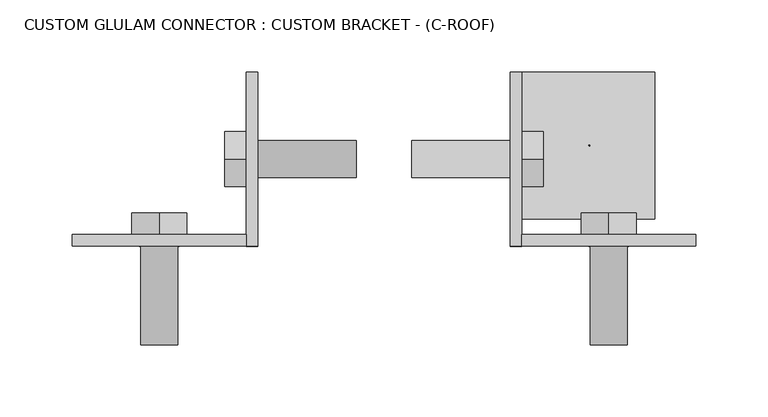
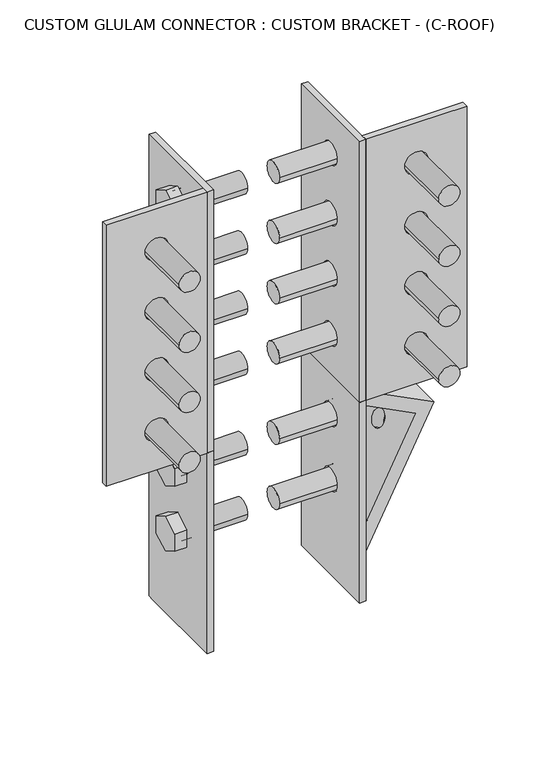
"""IFC4 building model written with IfcOpenShell, lengths in millimetres: fastener geometry, CUSTOM GLULAM CONNECTOR : CUSTOM BRACKET - (C-ROOF)."""

from ifc_helpers import new_model, si_unit, point, frame, frame_2d, origin, place, context, project, spatial, polyline, circle_curve, trimmed, segment, composite_curve, outline, extrude, source, transform, mapped, element, save
from ifc_brep_helpers import plane_surface, revolved_surface, advanced_brep


def custom_glulam_connector_custom_bracket_c_roof_8839ad80(model_context):
    return source(origin(), model_context, "Body", "SolidModel", [
        advanced_brep(
        [(-95.25, -60.325, 7.9375), (-87.3125, -60.325, 7.9375), (-87.3125, -60.325, 261.9375), (-95.25, -60.325, 261.9375), (-95.25, 60.325, 261.9375), (-87.3125, 60.325, 261.9375), (-87.3125, 60.325, 7.9375), (-95.25, 60.325, 7.9375), (-95.25, -13.890625, 128.5875), (-95.25, 13.890625, 128.5875), (-87.3125, 13.890625, 128.5875), (-87.3125, -13.890625, 128.5875), (-95.25, 52.3875, 7.9375), (-95.25, 52.3875, 261.9375), (-95.25, 13.890625, 211.1375), (-95.25, -13.890625, 211.1375), (-87.3125, -13.890625, 211.1375), (-87.3125, 13.890625, 211.1375)],
        [
            (0, 1),
            (1, 2),
            (2, 3),
            (3, 0),
            (4, 5),
            (5, 6),
            (6, 7),
            (7, 4),
            (8, 9, circle_curve(frame((-95.25, 0.0, 128.5875), z_axis=(-1.0, 0.0, 0.0), x_axis=(0.0, 1.0, 0.0)), 13.890625)),
            (9, 10),
            (10, 11, circle_curve(frame((-87.3125, 0.0, 128.5875), z_axis=(1.0, 0.0, 0.0), x_axis=(0.0, 1.0, 0.0)), 13.890625)),
            (11, 8),
            (7, 12),
            (12, 0),
            (3, 13),
            (13, 4),
            (8, 9, circle_curve(frame((-95.25, 0.0, 128.5875), z_axis=(1.0, 0.0, 0.0), x_axis=(0.0, 1.0, 0.0)), 13.890625)),
            (14, 15, circle_curve(frame((-95.25, 0.0, 211.1375), z_axis=(1.0, 0.0, 0.0), x_axis=(0.0, 1.0, 0.0)), 13.890625)),
            (15, 14, circle_curve(frame((-95.25, 0.0, 211.1375), z_axis=(1.0, 0.0, 0.0), x_axis=(0.0, 1.0, 0.0)), 13.890625)),
            (16, 17, circle_curve(frame((-87.3125, 0.0, 211.1375), z_axis=(1.0, 0.0, 0.0), x_axis=(0.0, 1.0, 0.0)), 13.890625)),
            (17, 14),
            (15, 16),
            (17, 16, circle_curve(frame((-87.3125, 0.0, 211.1375), z_axis=(1.0, 0.0, 0.0), x_axis=(0.0, 1.0, 0.0)), 13.890625)),
            (11, 10, circle_curve(frame((-87.3125, 0.0, 128.5875), z_axis=(1.0, 0.0, 0.0), x_axis=(0.0, 1.0, 0.0)), 13.890625)),
            (5, 2),
            (1, 6),
        ],
        [
            plane_surface(frame((-95.25, -60.325, 261.9375), z_axis=(0.0, -1.0, 0.0), x_axis=(1.0, 0.0, 0.0))),
            plane_surface(frame((-95.25, 60.325, 7.9375), z_axis=(0.0, 1.0, 0.0), x_axis=(1.0, 0.0, 0.0))),
            revolved_surface(polyline([(-95.25, 13.890625, 128.5875), (-87.3125, 13.890625, 128.5875)]), (-87.3125, 0.0, 128.5875), (-1.0, 0.0, 0.0)),
            plane_surface(frame((-95.25, -60.325, 261.9375), z_axis=(-1.0, 0.0, 0.0), x_axis=(0.0, -1.0, 0.0))),
            revolved_surface(polyline([(-95.25, 13.890625, 211.1375), (-87.3125, 13.890625, 211.1375)]), (-87.3125, 0.0, 211.1375), (-1.0, 0.0, 0.0)),
            plane_surface(frame((-87.3125, -60.325, 261.9375), z_axis=(1.0, 0.0, 0.0), x_axis=(0.0, 1.0, 0.0))),
            plane_surface(frame((-95.25, 60.325, 261.9375), z_axis=(0.0, 0.0, 1.0), x_axis=(1.0, 0.0, 0.0))),
            plane_surface(frame((-95.25, -60.325, 7.9375), z_axis=(0.0, 0.0, -1.0), x_axis=(1.0, 0.0, 0.0))),
        ],
        [
            (0, [[1, 2, 3, 4]]),
            (1, [[5, 6, 7, 8]]),
            (2, [[9, 10, 11, 12]]),
            (3, [[-8, 13, 14, -4, 15, 16], [-9, 17], [18, 19]]),
            (4, [[20, 21, -19, 22]]),
            (4, [[-18, -21, 23, -22]]),
            (2, [[24, -10, -17, -12]]),
            (5, [[25, -2, 26, -6], [-23, -20], [-11, -24]]),
            (6, [[-3, -25, -5, -16, -15]]),
            (7, [[-7, -26, -1, -14, -13]]),
        ],
    ),
        extrude(outline(polyline([(-19.05, 222.1360226), (0.0, 233.1345453), (19.05, 222.1360226), (19.05, 200.1389774), (0.0, 189.1404547), (-19.05, 200.1389774), (-19.05, 222.1360226)])), frame((-110.2320312, 0.0, 0.0), z_axis=(1.0, 0.0, 0.0), x_axis=(0.0, 1.0, 0.0)), (0.0, 0.0, 1.0), 14.9820312),
        extrude(outline(composite_curve([segment(trimmed(circle_curve(frame_2d((0.0, 211.1375)), 12.7), [point((-12.7, 211.1375))], [point((12.7, 211.1375))], False, "CARTESIAN"), True, "CONTINUOUS"), segment(trimmed(circle_curve(frame_2d((0.0, 211.1375)), 12.7), [point((12.7, 211.1375))], [point((-12.7, 211.1375))], False, "CARTESIAN"), True, "CONTINUOUS")], self_intersect=False)), frame((-95.25, 0.0, 0.0), z_axis=(1.0, 0.0, 0.0), x_axis=(0.0, 1.0, 0.0)), (0.0, 0.0, 1.0), 76.2),
        extrude(outline(polyline([(-19.05, 139.5860226), (0.0, 150.5845453), (19.05, 139.5860226), (19.05, 117.5889774), (0.0, 106.5904547), (-19.05, 117.5889774), (-19.05, 139.5860226)])), frame((-110.2320312, 0.0, 0.0), z_axis=(1.0, 0.0, 0.0), x_axis=(0.0, 1.0, 0.0)), (0.0, 0.0, 1.0), 14.9820312),
        extrude(outline(composite_curve([segment(trimmed(circle_curve(frame_2d((0.0, 128.5875)), 12.7), [point((-12.7, 128.5875))], [point((12.7, 128.5875))], False, "CARTESIAN"), True, "CONTINUOUS"), segment(trimmed(circle_curve(frame_2d((0.0, 128.5875)), 12.7), [point((12.7, 128.5875))], [point((-12.7, 128.5875))], False, "CARTESIAN"), True, "CONTINUOUS")], self_intersect=False)), frame((-95.25, 0.0, 0.0), z_axis=(1.0, 0.0, 0.0), x_axis=(0.0, 1.0, 0.0)), (0.0, 0.0, 1.0), 76.2),
        extrude(outline(polyline([(-19.05, 222.1360226), (0.0, 233.1345453), (19.05, 222.1360226), (19.05, 200.1389774), (0.0, 189.1404547), (-19.05, 200.1389774), (-19.05, 222.1360226)])), frame((-110.2320312, 0.0, 0.0), z_axis=(1.0, 0.0, 0.0), x_axis=(0.0, 1.0, 0.0)), (0.0, 0.0, 1.0), 14.9820312),
        extrude(outline(composite_curve([segment(trimmed(circle_curve(frame_2d((0.0, 211.1375)), 12.7), [point((-12.7, 211.1375))], [point((12.7, 211.1375))], False, "CARTESIAN"), True, "CONTINUOUS"), segment(trimmed(circle_curve(frame_2d((0.0, 211.1375)), 12.7), [point((12.7, 211.1375))], [point((-12.7, 211.1375))], False, "CARTESIAN"), True, "CONTINUOUS")], self_intersect=False)), frame((-95.25, 0.0, 0.0), z_axis=(1.0, 0.0, 0.0), x_axis=(0.0, 1.0, 0.0)), (0.0, 0.0, 1.0), 76.2),
        advanced_brep(
        [(95.25, -60.325, 7.9375), (95.25, -60.325, 261.9375), (87.3125, -60.325, 261.9375), (87.3125, -60.325, 7.9375), (95.25, 60.325, 261.9375), (95.25, 60.325, 7.9375), (87.3125, 60.325, 7.9375), (87.3125, 60.325, 261.9375), (95.25, -13.890625, 128.5875), (87.3125, -13.890625, 128.5875), (87.3125, 13.890625, 128.5875), (95.25, 13.890625, 128.5875), (95.25, 52.3875, 261.9375), (95.25, 52.3875, 7.9375), (95.25, 13.890625, 211.1375), (95.25, -13.890625, 211.1375), (87.3125, -13.890625, 211.1375), (87.3125, 13.890625, 211.1375)],
        [
            (0, 1),
            (1, 2),
            (2, 3),
            (3, 0),
            (4, 5),
            (5, 6),
            (6, 7),
            (7, 4),
            (8, 9),
            (9, 10, circle_curve(frame((87.3125, 0.0, 128.5875), z_axis=(-1.0, 0.0, 0.0), x_axis=(0.0, 1.0, 0.0)), 13.890625)),
            (10, 11),
            (11, 8, circle_curve(frame((95.25, 0.0, 128.5875), z_axis=(1.0, 0.0, 0.0), x_axis=(0.0, 1.0, 0.0)), 13.890625)),
            (4, 12),
            (12, 1),
            (0, 13),
            (13, 5),
            (14, 15, circle_curve(frame((95.25, 0.0, 211.1375), z_axis=(-1.0, 0.0, 0.0), x_axis=(0.0, 1.0, 0.0)), 13.890625)),
            (15, 14, circle_curve(frame((95.25, 0.0, 211.1375), z_axis=(-1.0, 0.0, 0.0), x_axis=(0.0, 1.0, 0.0)), 13.890625)),
            (11, 8, circle_curve(frame((95.25, 0.0, 128.5875), z_axis=(-1.0, 0.0, 0.0), x_axis=(0.0, 1.0, 0.0)), 13.890625)),
            (16, 15),
            (14, 17),
            (17, 16, circle_curve(frame((87.3125, 0.0, 211.1375), z_axis=(-1.0, 0.0, 0.0), x_axis=(0.0, 1.0, 0.0)), 13.890625)),
            (16, 17, circle_curve(frame((87.3125, 0.0, 211.1375), z_axis=(-1.0, 0.0, 0.0), x_axis=(0.0, 1.0, 0.0)), 13.890625)),
            (10, 9, circle_curve(frame((87.3125, 0.0, 128.5875), z_axis=(-1.0, 0.0, 0.0), x_axis=(0.0, 1.0, 0.0)), 13.890625)),
            (6, 3),
            (2, 7),
        ],
        [
            plane_surface(frame((95.25, -60.325, 261.9375), z_axis=(0.0, -1.0, 0.0), x_axis=(-1.0, 0.0, 0.0))),
            plane_surface(frame((95.25, 60.325, 7.9375), z_axis=(0.0, 1.0, 0.0), x_axis=(-1.0, 0.0, 0.0))),
            revolved_surface(polyline([(95.25, 13.890625, 128.5875), (87.3125, 13.890625, 128.5875)]), (87.3125, 0.0, 128.5875), (1.0, 0.0, 0.0)),
            plane_surface(frame((95.25, -60.325, 261.9375), z_axis=(1.0, 0.0, 0.0), x_axis=(0.0, -1.0, 0.0))),
            revolved_surface(polyline([(95.25, 13.890625, 211.1375), (87.3125, 13.890625, 211.1375)]), (87.3125, 0.0, 211.1375), (1.0, 0.0, 0.0)),
            plane_surface(frame((87.3125, -60.325, 261.9375), z_axis=(-1.0, 0.0, 0.0), x_axis=(0.0, 1.0, 0.0))),
            plane_surface(frame((95.25, 60.325, 261.9375), z_axis=(0.0, 0.0, 1.0), x_axis=(-1.0, 0.0, 0.0))),
            plane_surface(frame((95.25, -60.325, 7.9375), z_axis=(0.0, 0.0, -1.0), x_axis=(-1.0, 0.0, 0.0))),
        ],
        [
            (0, [[1, 2, 3, 4]]),
            (1, [[5, 6, 7, 8]]),
            (2, [[9, 10, 11, 12]]),
            (3, [[13, 14, -1, 15, 16, -5], [17, 18], [19, -12]]),
            (4, [[20, -17, 21, 22]]),
            (4, [[-20, 23, -21, -18]]),
            (2, [[-9, -19, -11, 24]]),
            (5, [[-7, 25, -3, 26], [-22, -23], [-24, -10]]),
            (6, [[-14, -13, -8, -26, -2]]),
            (7, [[-16, -15, -4, -25, -6]]),
        ],
    ),
        extrude(outline(polyline([(-19.05, 222.1360226), (0.0, 233.1345453), (19.05, 222.1360226), (19.05, 200.1389774), (0.0, 189.1404547), (-19.05, 200.1389774), (-19.05, 222.1360226)])), frame((95.25, 0.0, 0.0), z_axis=(1.0, 0.0, 0.0), x_axis=(0.0, 1.0, 0.0)), (0.0, 0.0, 1.0), 14.9820312),
        extrude(outline(composite_curve([segment(trimmed(circle_curve(frame_2d((0.0, 211.1375)), 12.7), [point((-12.7, 211.1375))], [point((12.7, 211.1375))], False, "CARTESIAN"), True, "CONTINUOUS"), segment(trimmed(circle_curve(frame_2d((0.0, 211.1375)), 12.7), [point((12.7, 211.1375))], [point((-12.7, 211.1375))], False, "CARTESIAN"), True, "CONTINUOUS")], self_intersect=False)), frame((19.05, 0.0, 0.0), z_axis=(1.0, 0.0, 0.0), x_axis=(0.0, 1.0, 0.0)), (0.0, 0.0, 1.0), 76.2),
        extrude(outline(polyline([(-19.05, 139.5860226), (0.0, 150.5845453), (19.05, 139.5860226), (19.05, 117.5889774), (0.0, 106.5904547), (-19.05, 117.5889774), (-19.05, 139.5860226)])), frame((95.25, 0.0, 0.0), z_axis=(1.0, 0.0, 0.0), x_axis=(0.0, 1.0, 0.0)), (0.0, 0.0, 1.0), 14.9820312),
        extrude(outline(composite_curve([segment(trimmed(circle_curve(frame_2d((0.0, 128.5875)), 12.7), [point((-12.7, 128.5875))], [point((12.7, 128.5875))], False, "CARTESIAN"), True, "CONTINUOUS"), segment(trimmed(circle_curve(frame_2d((0.0, 128.5875)), 12.7), [point((12.7, 128.5875))], [point((-12.7, 128.5875))], False, "CARTESIAN"), True, "CONTINUOUS")], self_intersect=False)), frame((19.05, 0.0, 0.0), z_axis=(1.0, 0.0, 0.0), x_axis=(0.0, 1.0, 0.0)), (0.0, 0.0, 1.0), 76.2),
        extrude(outline(polyline([(-19.05, 222.1360226), (0.0, 233.1345453), (19.05, 222.1360226), (19.05, 200.1389774), (0.0, 189.1404547), (-19.05, 200.1389774), (-19.05, 222.1360226)])), frame((95.25, 0.0, 0.0), z_axis=(1.0, 0.0, 0.0), x_axis=(0.0, 1.0, 0.0)), (0.0, 0.0, 1.0), 14.9820312),
        extrude(outline(composite_curve([segment(trimmed(circle_curve(frame_2d((0.0, 211.1375)), 12.7), [point((-12.7, 211.1375))], [point((12.7, 211.1375))], False, "CARTESIAN"), True, "CONTINUOUS"), segment(trimmed(circle_curve(frame_2d((0.0, 211.1375)), 12.7), [point((12.7, 211.1375))], [point((-12.7, 211.1375))], False, "CARTESIAN"), True, "CONTINUOUS")], self_intersect=False)), frame((19.05, 0.0, 0.0), z_axis=(1.0, 0.0, 0.0), x_axis=(0.0, 1.0, 0.0)), (0.0, 0.0, 1.0), 76.2),
        extrude(outline(polyline([(592.1375, -215.9), (261.9375, -215.9), (261.9375, -95.25), (592.1375, -95.25), (592.1375, -215.9)]), holes=[composite_curve([segment(trimmed(circle_curve(frame_2d((541.3375, -155.575)), 13.890625), [point((541.3375, -141.684375))], [point((541.3375, -169.465625))], True, "CARTESIAN"), True, "CONTINUOUS"), segment(trimmed(circle_curve(frame_2d((541.3375, -155.575)), 13.890625), [point((541.3375, -169.465625))], [point((541.3375, -141.684375))], True, "CARTESIAN"), True, "CONTINUOUS")], self_intersect=False), composite_curve([segment(trimmed(circle_curve(frame_2d((465.1375, -155.575)), 13.890625), [point((465.1375, -141.684375))], [point((465.1375, -169.465625))], True, "CARTESIAN"), True, "CONTINUOUS"), segment(trimmed(circle_curve(frame_2d((465.1375, -155.575)), 13.890625), [point((465.1375, -169.465625))], [point((465.1375, -141.684375))], True, "CARTESIAN"), True, "CONTINUOUS")], self_intersect=False), composite_curve([segment(trimmed(circle_curve(frame_2d((388.9375, -155.575)), 13.890625), [point((388.9375, -141.684375))], [point((388.9375, -169.465625))], True, "CARTESIAN"), True, "CONTINUOUS"), segment(trimmed(circle_curve(frame_2d((388.9375, -155.575)), 13.890625), [point((388.9375, -169.465625))], [point((388.9375, -141.684375))], True, "CARTESIAN"), True, "CONTINUOUS")], self_intersect=False), composite_curve([segment(trimmed(circle_curve(frame_2d((312.7375, -155.575)), 13.890625), [point((312.7375, -141.684375))], [point((312.7375, -169.465625))], True, "CARTESIAN"), True, "CONTINUOUS"), segment(trimmed(circle_curve(frame_2d((312.7375, -155.575)), 13.890625), [point((312.7375, -169.465625))], [point((312.7375, -141.684375))], True, "CARTESIAN"), True, "CONTINUOUS")], self_intersect=False)]), frame((0.0, -60.325, 0.0), z_axis=(0.0, 1.0, 0.0), x_axis=(0.0, 0.0, 1.0)), (0.0, 0.0, 1.0), 7.9375),
        extrude(outline(polyline([(552.3360226, -136.525), (563.3345453, -155.575), (552.3360226, -174.625), (530.3389774, -174.625), (519.3404547, -155.575), (530.3389774, -136.525), (552.3360226, -136.525)])), frame((0.0, -52.3875, 0.0), z_axis=(0.0, 1.0, 0.0), x_axis=(0.0, 0.0, 1.0)), (0.0, 0.0, 1.0), 14.9820312),
        extrude(outline(composite_curve([segment(trimmed(circle_curve(frame_2d((541.3375, -155.575)), 12.7), [point((541.3375, -142.875))], [point((541.3375, -168.275))], False, "CARTESIAN"), True, "CONTINUOUS"), segment(trimmed(circle_curve(frame_2d((541.3375, -155.575)), 12.7), [point((541.3375, -168.275))], [point((541.3375, -142.875))], False, "CARTESIAN"), True, "CONTINUOUS")], self_intersect=False)), frame((0.0, -128.5875, 0.0), z_axis=(0.0, 1.0, 0.0), x_axis=(0.0, 0.0, 1.0)), (0.0, 0.0, 1.0), 76.2),
        extrude(outline(polyline([(476.1360226, -136.525), (487.1345453, -155.575), (476.1360226, -174.625), (454.1389774, -174.625), (443.1404547, -155.575), (454.1389774, -136.525), (476.1360226, -136.525)])), frame((0.0, -52.3875, 0.0), z_axis=(0.0, 1.0, 0.0), x_axis=(0.0, 0.0, 1.0)), (0.0, 0.0, 1.0), 14.9820312),
        extrude(outline(composite_curve([segment(trimmed(circle_curve(frame_2d((465.1375, -155.575)), 12.7), [point((465.1375, -142.875))], [point((465.1375, -168.275))], False, "CARTESIAN"), True, "CONTINUOUS"), segment(trimmed(circle_curve(frame_2d((465.1375, -155.575)), 12.7), [point((465.1375, -168.275))], [point((465.1375, -142.875))], False, "CARTESIAN"), True, "CONTINUOUS")], self_intersect=False)), frame((0.0, -128.5875, 0.0), z_axis=(0.0, 1.0, 0.0), x_axis=(0.0, 0.0, 1.0)), (0.0, 0.0, 1.0), 76.2),
        extrude(outline(polyline([(552.3360226, -136.525), (563.3345453, -155.575), (552.3360226, -174.625), (530.3389774, -174.625), (519.3404547, -155.575), (530.3389774, -136.525), (552.3360226, -136.525)])), frame((0.0, -52.3875, 0.0), z_axis=(0.0, 1.0, 0.0), x_axis=(0.0, 0.0, 1.0)), (0.0, 0.0, 1.0), 14.9820312),
        extrude(outline(composite_curve([segment(trimmed(circle_curve(frame_2d((541.3375, -155.575)), 12.7), [point((541.3375, -142.875))], [point((541.3375, -168.275))], False, "CARTESIAN"), True, "CONTINUOUS"), segment(trimmed(circle_curve(frame_2d((541.3375, -155.575)), 12.7), [point((541.3375, -168.275))], [point((541.3375, -142.875))], False, "CARTESIAN"), True, "CONTINUOUS")], self_intersect=False)), frame((0.0, -128.5875, 0.0), z_axis=(0.0, 1.0, 0.0), x_axis=(0.0, 0.0, 1.0)), (0.0, 0.0, 1.0), 76.2),
        extrude(outline(polyline([(399.9360226, -136.525), (410.9345453, -155.575), (399.9360226, -174.625), (377.9389774, -174.625), (366.9404547, -155.575), (377.9389774, -136.525), (399.9360226, -136.525)])), frame((0.0, -52.3875, 0.0), z_axis=(0.0, 1.0, 0.0), x_axis=(0.0, 0.0, 1.0)), (0.0, 0.0, 1.0), 14.9820312),
        extrude(outline(composite_curve([segment(trimmed(circle_curve(frame_2d((388.9375, -155.575)), 12.7), [point((388.9375, -142.875))], [point((388.9375, -168.275))], False, "CARTESIAN"), True, "CONTINUOUS"), segment(trimmed(circle_curve(frame_2d((388.9375, -155.575)), 12.7), [point((388.9375, -168.275))], [point((388.9375, -142.875))], False, "CARTESIAN"), True, "CONTINUOUS")], self_intersect=False)), frame((0.0, -128.5875, 0.0), z_axis=(0.0, 1.0, 0.0), x_axis=(0.0, 0.0, 1.0)), (0.0, 0.0, 1.0), 76.2),
        extrude(outline(polyline([(323.7360226, -136.525), (334.7345453, -155.575), (323.7360226, -174.625), (301.7389774, -174.625), (290.7404547, -155.575), (301.7389774, -136.525), (323.7360226, -136.525)])), frame((0.0, -52.3875, 0.0), z_axis=(0.0, 1.0, 0.0), x_axis=(0.0, 0.0, 1.0)), (0.0, 0.0, 1.0), 14.9820312),
        extrude(outline(composite_curve([segment(trimmed(circle_curve(frame_2d((312.7375, -155.575)), 12.7), [point((312.7375, -142.875))], [point((312.7375, -168.275))], False, "CARTESIAN"), True, "CONTINUOUS"), segment(trimmed(circle_curve(frame_2d((312.7375, -155.575)), 12.7), [point((312.7375, -168.275))], [point((312.7375, -142.875))], False, "CARTESIAN"), True, "CONTINUOUS")], self_intersect=False)), frame((0.0, -128.5875, 0.0), z_axis=(0.0, 1.0, 0.0), x_axis=(0.0, 0.0, 1.0)), (0.0, 0.0, 1.0), 76.2),
        advanced_brep(
        [(-95.25, -60.325, 261.9375), (-87.3125, -60.325, 261.9375), (-87.3125, -60.325, 592.1375), (-95.25, -60.325, 592.1375), (-95.25, 60.325, 592.1375), (-87.3125, 60.325, 592.1375), (-87.3125, 60.325, 261.9375), (-95.25, 60.325, 261.9375), (-95.25, -13.890625, 465.1375), (-95.25, 13.890625, 465.1375), (-87.3125, 13.890625, 465.1375), (-87.3125, -13.890625, 465.1375), (-95.25, -52.3875, 261.9375), (-95.25, -52.3875, 592.1375), (-95.25, 13.890625, 541.3375), (-95.25, -13.890625, 541.3375), (-95.25, 13.890625, 388.9375), (-95.25, -13.890625, 388.9375), (-95.25, 13.890625, 312.7375), (-95.25, -13.890625, 312.7375), (-87.3125, -13.890625, 541.3375), (-87.3125, 13.890625, 541.3375), (-87.3125, -13.890625, 388.9375), (-87.3125, 13.890625, 388.9375), (-87.3125, -13.890625, 312.7375), (-87.3125, 13.890625, 312.7375)],
        [
            (0, 1),
            (1, 2),
            (2, 3),
            (3, 0),
            (4, 5),
            (5, 6),
            (6, 7),
            (7, 4),
            (8, 9, circle_curve(frame((-95.25, 0.0, 465.1375), z_axis=(-1.0, 0.0, 0.0), x_axis=(0.0, 1.0, 0.0)), 13.890625)),
            (9, 10),
            (10, 11, circle_curve(frame((-87.3125, 0.0, 465.1375), z_axis=(1.0, 0.0, 0.0), x_axis=(0.0, 1.0, 0.0)), 13.890625)),
            (11, 8),
            (7, 12),
            (12, 0),
            (3, 13),
            (13, 4),
            (8, 9, circle_curve(frame((-95.25, 0.0, 465.1375), z_axis=(1.0, 0.0, 0.0), x_axis=(0.0, 1.0, 0.0)), 13.890625)),
            (14, 15, circle_curve(frame((-95.25, 0.0, 541.3375), z_axis=(1.0, 0.0, 0.0), x_axis=(0.0, 1.0, 0.0)), 13.890625)),
            (15, 14, circle_curve(frame((-95.25, 0.0, 541.3375), z_axis=(1.0, 0.0, 0.0), x_axis=(0.0, 1.0, 0.0)), 13.890625)),
            (16, 17, circle_curve(frame((-95.25, 0.0, 388.9375), z_axis=(1.0, 0.0, 0.0), x_axis=(0.0, 1.0, 0.0)), 13.890625)),
            (17, 16, circle_curve(frame((-95.25, 0.0, 388.9375), z_axis=(1.0, 0.0, 0.0), x_axis=(0.0, 1.0, 0.0)), 13.890625)),
            (18, 19, circle_curve(frame((-95.25, 0.0, 312.7375), z_axis=(1.0, 0.0, 0.0), x_axis=(0.0, 1.0, 0.0)), 13.890625)),
            (19, 18, circle_curve(frame((-95.25, 0.0, 312.7375), z_axis=(1.0, 0.0, 0.0), x_axis=(0.0, 1.0, 0.0)), 13.890625)),
            (20, 21, circle_curve(frame((-87.3125, 0.0, 541.3375), z_axis=(1.0, 0.0, 0.0), x_axis=(0.0, 1.0, 0.0)), 13.890625)),
            (21, 14),
            (15, 20),
            (21, 20, circle_curve(frame((-87.3125, 0.0, 541.3375), z_axis=(1.0, 0.0, 0.0), x_axis=(0.0, 1.0, 0.0)), 13.890625)),
            (11, 10, circle_curve(frame((-87.3125, 0.0, 465.1375), z_axis=(1.0, 0.0, 0.0), x_axis=(0.0, 1.0, 0.0)), 13.890625)),
            (5, 2),
            (1, 6),
            (22, 23, circle_curve(frame((-87.3125, 0.0, 388.9375), z_axis=(-1.0, 0.0, 0.0), x_axis=(0.0, 1.0, 0.0)), 13.890625)),
            (23, 22, circle_curve(frame((-87.3125, 0.0, 388.9375), z_axis=(-1.0, 0.0, 0.0), x_axis=(0.0, 1.0, 0.0)), 13.890625)),
            (24, 25, circle_curve(frame((-87.3125, 0.0, 312.7375), z_axis=(-1.0, 0.0, 0.0), x_axis=(0.0, 1.0, 0.0)), 13.890625)),
            (25, 24, circle_curve(frame((-87.3125, 0.0, 312.7375), z_axis=(-1.0, 0.0, 0.0), x_axis=(0.0, 1.0, 0.0)), 13.890625)),
            (18, 25),
            (24, 19),
            (16, 23),
            (22, 17),
        ],
        [
            plane_surface(frame((-95.25, -60.325, 592.1375), z_axis=(0.0, -1.0, 0.0), x_axis=(1.0, 0.0, 0.0))),
            plane_surface(frame((-95.25, 60.325, 261.9375), z_axis=(0.0, 1.0, 0.0), x_axis=(1.0, 0.0, 0.0))),
            revolved_surface(polyline([(-95.25, 13.890625, 465.1375), (-87.3125, 13.890625, 465.1375)]), (-87.3125, 0.0, 465.1375), (-1.0, 0.0, 0.0)),
            plane_surface(frame((-95.25, -60.325, 592.1375), z_axis=(-1.0, 0.0, 0.0), x_axis=(0.0, -1.0, 0.0))),
            revolved_surface(polyline([(-95.25, 13.890625, 541.3375), (-87.3125, 13.890625, 541.3375)]), (-87.3125, 0.0, 541.3375), (-1.0, 0.0, 0.0)),
            plane_surface(frame((-87.3125, -60.325, 592.1375), z_axis=(1.0, 0.0, 0.0), x_axis=(0.0, 1.0, 0.0))),
            plane_surface(frame((-95.25, 60.325, 592.1375), z_axis=(0.0, 0.0, 1.0), x_axis=(1.0, 0.0, 0.0))),
            plane_surface(frame((-95.25, -60.325, 261.9375), z_axis=(0.0, 0.0, -1.0), x_axis=(1.0, 0.0, 0.0))),
            revolved_surface(polyline([(-95.25, 13.890625, 312.7375), (-87.3125, 13.890625, 312.7375)]), (-87.3125, 0.0, 312.7375), (-1.0, 0.0, 0.0)),
            revolved_surface(polyline([(-95.25, 13.890625, 388.9375), (-87.3125, 13.890625, 388.9375)]), (-87.3125, 0.0, 388.9375), (-1.0, 0.0, 0.0)),
        ],
        [
            (0, [[1, 2, 3, 4]]),
            (1, [[5, 6, 7, 8]]),
            (2, [[9, 10, 11, 12]]),
            (3, [[-8, 13, 14, -4, 15, 16], [-9, 17], [18, 19], [20, 21], [22, 23]]),
            (4, [[24, 25, -19, 26]]),
            (4, [[-18, -25, 27, -26]]),
            (2, [[28, -10, -17, -12]]),
            (5, [[29, -2, 30, -6], [-27, -24], [-11, -28], [31, 32], [33, 34]]),
            (6, [[-3, -29, -5, -16, -15]]),
            (7, [[-7, -30, -1, -14, -13]]),
            (8, [[-22, 35, -33, 36]]),
            (9, [[-20, 37, -31, 38]]),
            (8, [[-34, -35, -23, -36]]),
            (9, [[-32, -37, -21, -38]]),
        ],
    ),
        extrude(outline(polyline([(-19.05, 552.3360226), (0.0, 563.3345453), (19.05, 552.3360226), (19.05, 530.3389774), (0.0, 519.3404547), (-19.05, 530.3389774), (-19.05, 552.3360226)])), frame((-110.2320312, 0.0, 0.0), z_axis=(1.0, 0.0, 0.0), x_axis=(0.0, 1.0, 0.0)), (0.0, 0.0, 1.0), 14.9820312),
        extrude(outline(composite_curve([segment(trimmed(circle_curve(frame_2d((0.0, 541.3375)), 12.7), [point((-12.7, 541.3375))], [point((12.7, 541.3375))], False, "CARTESIAN"), True, "CONTINUOUS"), segment(trimmed(circle_curve(frame_2d((0.0, 541.3375)), 12.7), [point((12.7, 541.3375))], [point((-12.7, 541.3375))], False, "CARTESIAN"), True, "CONTINUOUS")], self_intersect=False)), frame((-95.25, 0.0, 0.0), z_axis=(1.0, 0.0, 0.0), x_axis=(0.0, 1.0, 0.0)), (0.0, 0.0, 1.0), 76.2),
        extrude(outline(polyline([(-19.05, 476.1360226), (0.0, 487.1345453), (19.05, 476.1360226), (19.05, 454.1389774), (0.0, 443.1404547), (-19.05, 454.1389774), (-19.05, 476.1360226)])), frame((-110.2320312, 0.0, 0.0), z_axis=(1.0, 0.0, 0.0), x_axis=(0.0, 1.0, 0.0)), (0.0, 0.0, 1.0), 14.9820312),
        extrude(outline(composite_curve([segment(trimmed(circle_curve(frame_2d((0.0, 465.1375)), 12.7), [point((-12.7, 465.1375))], [point((12.7, 465.1375))], False, "CARTESIAN"), True, "CONTINUOUS"), segment(trimmed(circle_curve(frame_2d((0.0, 465.1375)), 12.7), [point((12.7, 465.1375))], [point((-12.7, 465.1375))], False, "CARTESIAN"), True, "CONTINUOUS")], self_intersect=False)), frame((-95.25, 0.0, 0.0), z_axis=(1.0, 0.0, 0.0), x_axis=(0.0, 1.0, 0.0)), (0.0, 0.0, 1.0), 76.2),
        extrude(outline(polyline([(-19.05, 552.3360226), (0.0, 563.3345453), (19.05, 552.3360226), (19.05, 530.3389774), (0.0, 519.3404547), (-19.05, 530.3389774), (-19.05, 552.3360226)])), frame((-110.2320312, 0.0, 0.0), z_axis=(1.0, 0.0, 0.0), x_axis=(0.0, 1.0, 0.0)), (0.0, 0.0, 1.0), 14.9820312),
        extrude(outline(composite_curve([segment(trimmed(circle_curve(frame_2d((0.0, 541.3375)), 12.7), [point((-12.7, 541.3375))], [point((12.7, 541.3375))], False, "CARTESIAN"), True, "CONTINUOUS"), segment(trimmed(circle_curve(frame_2d((0.0, 541.3375)), 12.7), [point((12.7, 541.3375))], [point((-12.7, 541.3375))], False, "CARTESIAN"), True, "CONTINUOUS")], self_intersect=False)), frame((-95.25, 0.0, 0.0), z_axis=(1.0, 0.0, 0.0), x_axis=(0.0, 1.0, 0.0)), (0.0, 0.0, 1.0), 76.2),
        extrude(outline(polyline([(-19.05, 399.9360226), (0.0, 410.9345453), (19.05, 399.9360226), (19.05, 377.9389774), (0.0, 366.9404547), (-19.05, 377.9389774), (-19.05, 399.9360226)])), frame((-110.2320312, 0.0, 0.0), z_axis=(1.0, 0.0, 0.0), x_axis=(0.0, 1.0, 0.0)), (0.0, 0.0, 1.0), 14.9820312),
        extrude(outline(composite_curve([segment(trimmed(circle_curve(frame_2d((0.0, 388.9375)), 12.7), [point((-12.7, 388.9375))], [point((12.7, 388.9375))], False, "CARTESIAN"), True, "CONTINUOUS"), segment(trimmed(circle_curve(frame_2d((0.0, 388.9375)), 12.7), [point((12.7, 388.9375))], [point((-12.7, 388.9375))], False, "CARTESIAN"), True, "CONTINUOUS")], self_intersect=False)), frame((-95.25, 0.0, 0.0), z_axis=(1.0, 0.0, 0.0), x_axis=(0.0, 1.0, 0.0)), (0.0, 0.0, 1.0), 76.2),
        extrude(outline(polyline([(-19.05, 323.7360226), (0.0, 334.7345453), (19.05, 323.7360226), (19.05, 301.7389774), (0.0, 290.7404547), (-19.05, 301.7389774), (-19.05, 323.7360226)])), frame((-110.2320312, 0.0, 0.0), z_axis=(1.0, 0.0, 0.0), x_axis=(0.0, 1.0, 0.0)), (0.0, 0.0, 1.0), 14.9820312),
        extrude(outline(composite_curve([segment(trimmed(circle_curve(frame_2d((0.0, 312.7375)), 12.7), [point((-12.7, 312.7375))], [point((12.7, 312.7375))], False, "CARTESIAN"), True, "CONTINUOUS"), segment(trimmed(circle_curve(frame_2d((0.0, 312.7375)), 12.7), [point((12.7, 312.7375))], [point((-12.7, 312.7375))], False, "CARTESIAN"), True, "CONTINUOUS")], self_intersect=False)), frame((-95.25, 0.0, 0.0), z_axis=(1.0, 0.0, 0.0), x_axis=(0.0, 1.0, 0.0)), (0.0, 0.0, 1.0), 76.2),
        extrude(outline(polyline([(592.1375, 215.9), (592.1375, 95.25), (261.9375, 95.25), (261.9375, 215.9), (592.1375, 215.9)]), holes=[composite_curve([segment(trimmed(circle_curve(frame_2d((541.3375, 155.575)), 13.890625), [point((541.3375, 141.684375))], [point((541.3375, 169.465625))], True, "CARTESIAN"), True, "CONTINUOUS"), segment(trimmed(circle_curve(frame_2d((541.3375, 155.575)), 13.890625), [point((541.3375, 169.465625))], [point((541.3375, 141.684375))], True, "CARTESIAN"), True, "CONTINUOUS")], self_intersect=False), composite_curve([segment(trimmed(circle_curve(frame_2d((465.1375, 155.575)), 13.890625), [point((465.1375, 141.684375))], [point((465.1375, 169.465625))], True, "CARTESIAN"), True, "CONTINUOUS"), segment(trimmed(circle_curve(frame_2d((465.1375, 155.575)), 13.890625), [point((465.1375, 169.465625))], [point((465.1375, 141.684375))], True, "CARTESIAN"), True, "CONTINUOUS")], self_intersect=False), composite_curve([segment(trimmed(circle_curve(frame_2d((388.9375, 155.575)), 13.890625), [point((388.9375, 141.684375))], [point((388.9375, 169.465625))], True, "CARTESIAN"), True, "CONTINUOUS"), segment(trimmed(circle_curve(frame_2d((388.9375, 155.575)), 13.890625), [point((388.9375, 169.465625))], [point((388.9375, 141.684375))], True, "CARTESIAN"), True, "CONTINUOUS")], self_intersect=False), composite_curve([segment(trimmed(circle_curve(frame_2d((312.7375, 155.575)), 13.890625), [point((312.7375, 141.684375))], [point((312.7375, 169.465625))], True, "CARTESIAN"), True, "CONTINUOUS"), segment(trimmed(circle_curve(frame_2d((312.7375, 155.575)), 13.890625), [point((312.7375, 169.465625))], [point((312.7375, 141.684375))], True, "CARTESIAN"), True, "CONTINUOUS")], self_intersect=False)]), frame((0.0, -60.325, 0.0), z_axis=(0.0, 1.0, 0.0), x_axis=(0.0, 0.0, 1.0)), (0.0, 0.0, 1.0), 7.9375),
        extrude(outline(polyline([(552.3360226, 136.525), (530.3389774, 136.525), (519.3404547, 155.575), (530.3389774, 174.625), (552.3360226, 174.625), (563.3345453, 155.575), (552.3360226, 136.525)])), frame((0.0, -52.3875, 0.0), z_axis=(0.0, 1.0, 0.0), x_axis=(0.0, 0.0, 1.0)), (0.0, 0.0, 1.0), 14.9820312),
        extrude(outline(composite_curve([segment(trimmed(circle_curve(frame_2d((541.3375, 155.575)), 12.7), [point((541.3375, 142.875))], [point((541.3375, 168.275))], False, "CARTESIAN"), True, "CONTINUOUS"), segment(trimmed(circle_curve(frame_2d((541.3375, 155.575)), 12.7), [point((541.3375, 168.275))], [point((541.3375, 142.875))], False, "CARTESIAN"), True, "CONTINUOUS")], self_intersect=False)), frame((0.0, -128.5875, 0.0), z_axis=(0.0, 1.0, 0.0), x_axis=(0.0, 0.0, 1.0)), (0.0, 0.0, 1.0), 76.2),
        extrude(outline(polyline([(476.1360226, 136.525), (454.1389774, 136.525), (443.1404547, 155.575), (454.1389774, 174.625), (476.1360226, 174.625), (487.1345453, 155.575), (476.1360226, 136.525)])), frame((0.0, -52.3875, 0.0), z_axis=(0.0, 1.0, 0.0), x_axis=(0.0, 0.0, 1.0)), (0.0, 0.0, 1.0), 14.9820312),
        extrude(outline(composite_curve([segment(trimmed(circle_curve(frame_2d((465.1375, 155.575)), 12.7), [point((465.1375, 142.875))], [point((465.1375, 168.275))], False, "CARTESIAN"), True, "CONTINUOUS"), segment(trimmed(circle_curve(frame_2d((465.1375, 155.575)), 12.7), [point((465.1375, 168.275))], [point((465.1375, 142.875))], False, "CARTESIAN"), True, "CONTINUOUS")], self_intersect=False)), frame((0.0, -128.5875, 0.0), z_axis=(0.0, 1.0, 0.0), x_axis=(0.0, 0.0, 1.0)), (0.0, 0.0, 1.0), 76.2),
        extrude(outline(polyline([(552.3360226, 136.525), (530.3389774, 136.525), (519.3404547, 155.575), (530.3389774, 174.625), (552.3360226, 174.625), (563.3345453, 155.575), (552.3360226, 136.525)])), frame((0.0, -52.3875, 0.0), z_axis=(0.0, 1.0, 0.0), x_axis=(0.0, 0.0, 1.0)), (0.0, 0.0, 1.0), 14.9820312),
        extrude(outline(composite_curve([segment(trimmed(circle_curve(frame_2d((541.3375, 155.575)), 12.7), [point((541.3375, 142.875))], [point((541.3375, 168.275))], False, "CARTESIAN"), True, "CONTINUOUS"), segment(trimmed(circle_curve(frame_2d((541.3375, 155.575)), 12.7), [point((541.3375, 168.275))], [point((541.3375, 142.875))], False, "CARTESIAN"), True, "CONTINUOUS")], self_intersect=False)), frame((0.0, -128.5875, 0.0), z_axis=(0.0, 1.0, 0.0), x_axis=(0.0, 0.0, 1.0)), (0.0, 0.0, 1.0), 76.2),
        extrude(outline(polyline([(399.9360226, 136.525), (377.9389774, 136.525), (366.9404547, 155.575), (377.9389774, 174.625), (399.9360226, 174.625), (410.9345453, 155.575), (399.9360226, 136.525)])), frame((0.0, -52.3875, 0.0), z_axis=(0.0, 1.0, 0.0), x_axis=(0.0, 0.0, 1.0)), (0.0, 0.0, 1.0), 14.9820312),
        extrude(outline(composite_curve([segment(trimmed(circle_curve(frame_2d((388.9375, 155.575)), 12.7), [point((388.9375, 142.875))], [point((388.9375, 168.275))], False, "CARTESIAN"), True, "CONTINUOUS"), segment(trimmed(circle_curve(frame_2d((388.9375, 155.575)), 12.7), [point((388.9375, 168.275))], [point((388.9375, 142.875))], False, "CARTESIAN"), True, "CONTINUOUS")], self_intersect=False)), frame((0.0, -128.5875, 0.0), z_axis=(0.0, 1.0, 0.0), x_axis=(0.0, 0.0, 1.0)), (0.0, 0.0, 1.0), 76.2),
        extrude(outline(polyline([(323.7360226, 136.525), (301.7389774, 136.525), (290.7404547, 155.575), (301.7389774, 174.625), (323.7360226, 174.625), (334.7345453, 155.575), (323.7360226, 136.525)])), frame((0.0, -52.3875, 0.0), z_axis=(0.0, 1.0, 0.0), x_axis=(0.0, 0.0, 1.0)), (0.0, 0.0, 1.0), 14.9820312),
        extrude(outline(composite_curve([segment(trimmed(circle_curve(frame_2d((312.7375, 155.575)), 12.7), [point((312.7375, 142.875))], [point((312.7375, 168.275))], False, "CARTESIAN"), True, "CONTINUOUS"), segment(trimmed(circle_curve(frame_2d((312.7375, 155.575)), 12.7), [point((312.7375, 168.275))], [point((312.7375, 142.875))], False, "CARTESIAN"), True, "CONTINUOUS")], self_intersect=False)), frame((0.0, -128.5875, 0.0), z_axis=(0.0, 1.0, 0.0), x_axis=(0.0, 0.0, 1.0)), (0.0, 0.0, 1.0), 76.2),
        advanced_brep(
        [(95.25, -60.325, 261.9375), (95.25, -60.325, 592.1375), (87.3125, -60.325, 592.1375), (87.3125, -60.325, 261.9375), (95.25, 60.325, 592.1375), (95.25, 60.325, 261.9375), (87.3125, 60.325, 261.9375), (87.3125, 60.325, 592.1375), (95.25, -13.890625, 465.1375), (87.3125, -13.890625, 465.1375), (87.3125, 13.890625, 465.1375), (95.25, 13.890625, 465.1375), (95.25, -52.3875, 592.1375), (95.25, -52.3875, 261.9375), (95.25, 13.890625, 541.3375), (95.25, -13.890625, 541.3375), (95.25, 13.890625, 312.7375), (95.25, -13.890625, 312.7375), (95.25, 13.890625, 388.9375), (95.25, -13.890625, 388.9375), (87.3125, -13.890625, 541.3375), (87.3125, 13.890625, 541.3375), (87.3125, -13.890625, 388.9375), (87.3125, 13.890625, 388.9375), (87.3125, -13.890625, 312.7375), (87.3125, 13.890625, 312.7375)],
        [
            (0, 1),
            (1, 2),
            (2, 3),
            (3, 0),
            (4, 5),
            (5, 6),
            (6, 7),
            (7, 4),
            (8, 9),
            (9, 10, circle_curve(frame((87.3125, 0.0, 465.1375), z_axis=(-1.0, 0.0, 0.0), x_axis=(0.0, 1.0, 0.0)), 13.890625)),
            (10, 11),
            (11, 8, circle_curve(frame((95.25, 0.0, 465.1375), z_axis=(1.0, 0.0, 0.0), x_axis=(0.0, 1.0, 0.0)), 13.890625)),
            (4, 12),
            (12, 1),
            (0, 13),
            (13, 5),
            (14, 15, circle_curve(frame((95.25, 0.0, 541.3375), z_axis=(-1.0, 0.0, 0.0), x_axis=(0.0, 1.0, 0.0)), 13.890625)),
            (15, 14, circle_curve(frame((95.25, 0.0, 541.3375), z_axis=(-1.0, 0.0, 0.0), x_axis=(0.0, 1.0, 0.0)), 13.890625)),
            (11, 8, circle_curve(frame((95.25, 0.0, 465.1375), z_axis=(-1.0, 0.0, 0.0), x_axis=(0.0, 1.0, 0.0)), 13.890625)),
            (16, 17, circle_curve(frame((95.25, 0.0, 312.7375), z_axis=(-1.0, 0.0, 0.0), x_axis=(0.0, 1.0, 0.0)), 13.890625)),
            (17, 16, circle_curve(frame((95.25, 0.0, 312.7375), z_axis=(-1.0, 0.0, 0.0), x_axis=(0.0, 1.0, 0.0)), 13.890625)),
            (18, 19, circle_curve(frame((95.25, 0.0, 388.9375), z_axis=(-1.0, 0.0, 0.0), x_axis=(0.0, 1.0, 0.0)), 13.890625)),
            (19, 18, circle_curve(frame((95.25, 0.0, 388.9375), z_axis=(-1.0, 0.0, 0.0), x_axis=(0.0, 1.0, 0.0)), 13.890625)),
            (20, 15),
            (14, 21),
            (21, 20, circle_curve(frame((87.3125, 0.0, 541.3375), z_axis=(-1.0, 0.0, 0.0), x_axis=(0.0, 1.0, 0.0)), 13.890625)),
            (20, 21, circle_curve(frame((87.3125, 0.0, 541.3375), z_axis=(-1.0, 0.0, 0.0), x_axis=(0.0, 1.0, 0.0)), 13.890625)),
            (10, 9, circle_curve(frame((87.3125, 0.0, 465.1375), z_axis=(-1.0, 0.0, 0.0), x_axis=(0.0, 1.0, 0.0)), 13.890625)),
            (6, 3),
            (2, 7),
            (22, 23, circle_curve(frame((87.3125, 0.0, 388.9375), z_axis=(1.0, 0.0, 0.0), x_axis=(0.0, 1.0, 0.0)), 13.890625)),
            (23, 22, circle_curve(frame((87.3125, 0.0, 388.9375), z_axis=(1.0, 0.0, 0.0), x_axis=(0.0, 1.0, 0.0)), 13.890625)),
            (24, 25, circle_curve(frame((87.3125, 0.0, 312.7375), z_axis=(1.0, 0.0, 0.0), x_axis=(0.0, 1.0, 0.0)), 13.890625)),
            (25, 24, circle_curve(frame((87.3125, 0.0, 312.7375), z_axis=(1.0, 0.0, 0.0), x_axis=(0.0, 1.0, 0.0)), 13.890625)),
            (17, 24),
            (25, 16),
            (19, 22),
            (23, 18),
        ],
        [
            plane_surface(frame((95.25, -60.325, 592.1375), z_axis=(0.0, -1.0, 0.0), x_axis=(-1.0, 0.0, 0.0))),
            plane_surface(frame((95.25, 60.325, 261.9375), z_axis=(0.0, 1.0, 0.0), x_axis=(-1.0, 0.0, 0.0))),
            revolved_surface(polyline([(95.25, 13.890625, 465.1375), (87.3125, 13.890625, 465.1375)]), (87.3125, 0.0, 465.1375), (1.0, 0.0, 0.0)),
            plane_surface(frame((95.25, -60.325, 592.1375), z_axis=(1.0, 0.0, 0.0), x_axis=(0.0, -1.0, 0.0))),
            revolved_surface(polyline([(95.25, 13.890625, 541.3375), (87.3125, 13.890625, 541.3375)]), (87.3125, 0.0, 541.3375), (1.0, 0.0, 0.0)),
            plane_surface(frame((87.3125, -60.325, 592.1375), z_axis=(-1.0, 0.0, 0.0), x_axis=(0.0, 1.0, 0.0))),
            plane_surface(frame((95.25, 60.325, 592.1375), z_axis=(0.0, 0.0, 1.0), x_axis=(-1.0, 0.0, 0.0))),
            plane_surface(frame((95.25, -60.325, 261.9375), z_axis=(0.0, 0.0, -1.0), x_axis=(-1.0, 0.0, 0.0))),
            revolved_surface(polyline([(95.25, 13.890625, 312.7375), (87.3125, 13.890625, 312.7375)]), (87.3125, 0.0, 312.7375), (1.0, 0.0, 0.0)),
            revolved_surface(polyline([(95.25, 13.890625, 388.9375), (87.3125, 13.890625, 388.9375)]), (87.3125, 0.0, 388.9375), (1.0, 0.0, 0.0)),
        ],
        [
            (0, [[1, 2, 3, 4]]),
            (1, [[5, 6, 7, 8]]),
            (2, [[9, 10, 11, 12]]),
            (3, [[13, 14, -1, 15, 16, -5], [17, 18], [19, -12], [20, 21], [22, 23]]),
            (4, [[24, -17, 25, 26]]),
            (4, [[-24, 27, -25, -18]]),
            (2, [[-9, -19, -11, 28]]),
            (5, [[-7, 29, -3, 30], [-26, -27], [-28, -10], [31, 32], [33, 34]]),
            (6, [[-14, -13, -8, -30, -2]]),
            (7, [[-16, -15, -4, -29, -6]]),
            (8, [[35, -34, 36, -21]]),
            (9, [[37, -32, 38, -23]]),
            (8, [[-35, -20, -36, -33]]),
            (9, [[-37, -22, -38, -31]]),
        ],
    ),
        extrude(outline(polyline([(-19.05, 552.3360226), (0.0, 563.3345453), (19.05, 552.3360226), (19.05, 530.3389774), (0.0, 519.3404547), (-19.05, 530.3389774), (-19.05, 552.3360226)])), frame((95.25, 0.0, 0.0), z_axis=(1.0, 0.0, 0.0), x_axis=(0.0, 1.0, 0.0)), (0.0, 0.0, 1.0), 14.9820312),
        extrude(outline(composite_curve([segment(trimmed(circle_curve(frame_2d((0.0, 541.3375)), 12.7), [point((-12.7, 541.3375))], [point((12.7, 541.3375))], False, "CARTESIAN"), True, "CONTINUOUS"), segment(trimmed(circle_curve(frame_2d((0.0, 541.3375)), 12.7), [point((12.7, 541.3375))], [point((-12.7, 541.3375))], False, "CARTESIAN"), True, "CONTINUOUS")], self_intersect=False)), frame((19.05, 0.0, 0.0), z_axis=(1.0, 0.0, 0.0), x_axis=(0.0, 1.0, 0.0)), (0.0, 0.0, 1.0), 76.2),
        extrude(outline(polyline([(-19.05, 476.1360226), (0.0, 487.1345453), (19.05, 476.1360226), (19.05, 454.1389774), (0.0, 443.1404547), (-19.05, 454.1389774), (-19.05, 476.1360226)])), frame((95.25, 0.0, 0.0), z_axis=(1.0, 0.0, 0.0), x_axis=(0.0, 1.0, 0.0)), (0.0, 0.0, 1.0), 14.9820312),
        extrude(outline(composite_curve([segment(trimmed(circle_curve(frame_2d((0.0, 465.1375)), 12.7), [point((-12.7, 465.1375))], [point((12.7, 465.1375))], False, "CARTESIAN"), True, "CONTINUOUS"), segment(trimmed(circle_curve(frame_2d((0.0, 465.1375)), 12.7), [point((12.7, 465.1375))], [point((-12.7, 465.1375))], False, "CARTESIAN"), True, "CONTINUOUS")], self_intersect=False)), frame((19.05, 0.0, 0.0), z_axis=(1.0, 0.0, 0.0), x_axis=(0.0, 1.0, 0.0)), (0.0, 0.0, 1.0), 76.2),
        extrude(outline(polyline([(-19.05, 552.3360226), (0.0, 563.3345453), (19.05, 552.3360226), (19.05, 530.3389774), (0.0, 519.3404547), (-19.05, 530.3389774), (-19.05, 552.3360226)])), frame((95.25, 0.0, 0.0), z_axis=(1.0, 0.0, 0.0), x_axis=(0.0, 1.0, 0.0)), (0.0, 0.0, 1.0), 14.9820312),
        extrude(outline(composite_curve([segment(trimmed(circle_curve(frame_2d((0.0, 541.3375)), 12.7), [point((-12.7, 541.3375))], [point((12.7, 541.3375))], False, "CARTESIAN"), True, "CONTINUOUS"), segment(trimmed(circle_curve(frame_2d((0.0, 541.3375)), 12.7), [point((12.7, 541.3375))], [point((-12.7, 541.3375))], False, "CARTESIAN"), True, "CONTINUOUS")], self_intersect=False)), frame((19.05, 0.0, 0.0), z_axis=(1.0, 0.0, 0.0), x_axis=(0.0, 1.0, 0.0)), (0.0, 0.0, 1.0), 76.2),
        extrude(outline(polyline([(-19.05, 399.9360226), (0.0, 410.9345453), (19.05, 399.9360226), (19.05, 377.9389774), (0.0, 366.9404547), (-19.05, 377.9389774), (-19.05, 399.9360226)])), frame((95.25, 0.0, 0.0), z_axis=(1.0, 0.0, 0.0), x_axis=(0.0, 1.0, 0.0)), (0.0, 0.0, 1.0), 14.9820312),
        extrude(outline(composite_curve([segment(trimmed(circle_curve(frame_2d((0.0, 388.9375)), 12.7), [point((-12.7, 388.9375))], [point((12.7, 388.9375))], False, "CARTESIAN"), True, "CONTINUOUS"), segment(trimmed(circle_curve(frame_2d((0.0, 388.9375)), 12.7), [point((12.7, 388.9375))], [point((-12.7, 388.9375))], False, "CARTESIAN"), True, "CONTINUOUS")], self_intersect=False)), frame((19.05, 0.0, 0.0), z_axis=(1.0, 0.0, 0.0), x_axis=(0.0, 1.0, 0.0)), (0.0, 0.0, 1.0), 76.2),
        extrude(outline(polyline([(-19.05, 323.7360226), (0.0, 334.7345453), (19.05, 323.7360226), (19.05, 301.7389774), (0.0, 290.7404547), (-19.05, 301.7389774), (-19.05, 323.7360226)])), frame((95.25, 0.0, 0.0), z_axis=(1.0, 0.0, 0.0), x_axis=(0.0, 1.0, 0.0)), (0.0, 0.0, 1.0), 14.9820312),
        extrude(outline(composite_curve([segment(trimmed(circle_curve(frame_2d((0.0, 312.7375)), 12.7), [point((-12.7, 312.7375))], [point((12.7, 312.7375))], False, "CARTESIAN"), True, "CONTINUOUS"), segment(trimmed(circle_curve(frame_2d((0.0, 312.7375)), 12.7), [point((12.7, 312.7375))], [point((-12.7, 312.7375))], False, "CARTESIAN"), True, "CONTINUOUS")], self_intersect=False)), frame((19.05, 0.0, 0.0), z_axis=(1.0, 0.0, 0.0), x_axis=(0.0, 1.0, 0.0)), (0.0, 0.0, 1.0), 76.2),
        advanced_brep(
        [(187.5008695, -41.275, 215.9775257), (95.25, -41.275, 262.9816915), (95.25, -41.275, 245.1647625), (166.1490418, -41.275, 209.0398963), (95.25, -41.275, 69.8926921), (95.25, -41.275, 34.925), (187.5008695, 60.325, 215.9775257), (95.25, 60.325, 34.925), (95.25, 60.325, 69.8926921), (166.1490418, 60.325, 209.0398963), (95.25, 60.325, 245.1647625), (95.25, 60.325, 262.9816915), (142.5913563, 9.525, 238.8600656), (141.8841199, 9.525, 239.2204206), (134.6770207, 9.525, 225.075692), (135.3842571, 9.525, 224.7153371), (155.1582155, 9.525, 187.4691853), (145.4286316, 9.525, 168.3738017), (159.5733602, 9.525, 161.1667025), (169.3029441, 9.525, 180.2620861)],
        [
            (0, 1),
            (1, 2),
            (2, 3),
            (3, 4),
            (4, 5),
            (5, 0),
            (6, 7),
            (7, 8),
            (8, 9),
            (9, 10),
            (10, 11),
            (11, 6),
            (0, 6),
            (11, 1),
            (12, 13, circle_curve(frame((142.2377381, 9.525, 239.0402431), z_axis=(-0.45399049973954914, 0.0, -0.8910065241883667), x_axis=(-0.8910065241883667, 0.0, 0.45399049973954914)), 0.396875)),
            (13, 12, circle_curve(frame((142.2377381, 9.525, 239.0402431), z_axis=(-0.45399049973954914, 0.0, -0.8910065241883667), x_axis=(-0.8910065241883667, 0.0, 0.45399049973954914)), 0.396875)),
            (10, 2),
            (9, 3),
            (14, 15, circle_curve(frame((135.0306389, 9.525, 224.8955145), z_axis=(0.45399049973954914, 0.0, 0.8910065241883667), x_axis=(-0.8910065241883667, 0.0, 0.45399049973954914)), 0.396875)),
            (15, 14, circle_curve(frame((135.0306389, 9.525, 224.8955145), z_axis=(0.45399049973954914, 0.0, 0.8910065241883667), x_axis=(-0.8910065241883667, 0.0, 0.45399049973954914)), 0.396875)),
            (8, 4),
            (16, 17, circle_curve(frame((150.2934236, 9.525, 177.9214935), z_axis=(0.891006524188366, 0.0, -0.45399049973955063), x_axis=(0.45399049973955063, 0.0, 0.891006524188366)), 10.715625)),
            (17, 16, circle_curve(frame((150.2934236, 9.525, 177.9214935), z_axis=(0.891006524188366, 0.0, -0.45399049973955063), x_axis=(0.45399049973955063, 0.0, 0.891006524188366)), 10.715625)),
            (7, 5),
            (18, 19, circle_curve(frame((164.4381522, 9.525, 170.7143943), z_axis=(-0.891006524188366, 0.0, 0.45399049973955063), x_axis=(0.45399049973955063, 0.0, 0.891006524188366)), 10.715625)),
            (19, 18, circle_curve(frame((164.4381522, 9.525, 170.7143943), z_axis=(-0.891006524188366, 0.0, 0.45399049973955063), x_axis=(0.45399049973955063, 0.0, 0.891006524188366)), 10.715625)),
            (12, 15),
            (14, 13),
            (18, 17),
            (16, 19),
        ],
        [
            plane_surface(frame((95.25, -41.275, 262.9816915), z_axis=(0.0, -1.0, 0.0), x_axis=(-0.8910065241883667, 0.0, 0.45399049973954914))),
            plane_surface(frame((95.25, 60.325, 262.9816915), z_axis=(0.0, 1.0, 0.0), x_axis=(0.8910065241883667, 0.0, -0.45399049973954914))),
            plane_surface(frame((187.5008695, -41.275, 215.9775257), z_axis=(0.45399049973954914, 0.0, 0.8910065241883667), x_axis=(0.0, 1.0, 0.0))),
            plane_surface(frame((95.25, -41.275, 262.9816915), z_axis=(-1.0, 0.0, 0.0), x_axis=(0.0, 1.0, 0.0))),
            plane_surface(frame((95.25, -41.275, 245.1647625), z_axis=(-0.4539904997395493, 0.0, -0.8910065241883667), x_axis=(0.0, 1.0, 0.0))),
            plane_surface(frame((166.1490418, -41.275, 209.0398963), z_axis=(-0.891006524188366, 0.0, 0.4539904997395506), x_axis=(0.0, 1.0, 0.0))),
            plane_surface(frame((95.25, -41.275, 69.8926921), z_axis=(-1.0, 0.0, 0.0), x_axis=(0.0, 1.0, 0.0))),
            plane_surface(frame((95.25, -41.275, 34.925), z_axis=(0.891006524188366, 0.0, -0.45399049973955063), x_axis=(0.0, 1.0, 0.0))),
            revolved_surface(polyline([(134.67702068738646, 9.525, 225.07569197873133), (141.88411989691585, 9.525, 239.22042060157148)]), (142.2377381, 9.525, 239.0402431), (-0.45399049973954914, 0.0, -0.8910065241883667)),
            revolved_surface(polyline([(155.1582155034376, 9.525, 187.4691853067466), (169.30294414877162, 9.525, 180.26208608575598)]), (164.4381522, 9.525, 170.7143943), (-0.891006524188366, 0.0, 0.45399049973955063)),
        ],
        [
            (0, [[1, 2, 3, 4, 5, 6]]),
            (1, [[7, 8, 9, 10, 11, 12]]),
            (2, [[-1, 13, -12, 14], [15, 16]]),
            (3, [[-2, -14, -11, 17]]),
            (4, [[-3, -17, -10, 18], [19, 20]]),
            (5, [[-4, -18, -9, 21], [22, 23]]),
            (6, [[-5, -21, -8, 24]]),
            (7, [[-6, -24, -7, -13], [25, 26]]),
            (8, [[27, -19, 28, -15]]),
            (8, [[-27, -16, -28, -20]]),
            (9, [[29, -22, 30, -25]]),
            (9, [[-29, -26, -30, -23]]),
        ],
    ),
    ])


if __name__ == "__main__":
    model = new_model("IFC4")
    model_context = context("Model", 3, world=origin())
    ifc_project = project(units=[si_unit("LENGTHUNIT", "METRE", prefix="MILLI")], contexts=[model_context])
    site = spatial("IfcSite", under=ifc_project)
    building = spatial("IfcBuilding", under=site)
    placement = place(None, origin())
    custom_glulam_connector_custom_bracket_c_roof_shape = custom_glulam_connector_custom_bracket_c_roof_8839ad80(model_context)
    element("IfcFastener", 1, ObjectType="CUSTOM GLULAM CONNECTOR : CUSTOM BRACKET - (C-ROOF)", at=placement, inside=building, context=model_context, shape_type="MappedRepresentation", body=[
        mapped(custom_glulam_connector_custom_bracket_c_roof_shape, transform((0.0, 0.0, 0.0), x_axis=(1.0, 0.0, 0.0), y_axis=(0.0, 1.0, 0.0), z_axis=(0.0, 0.0, 1.0))),
    ])
    save(model, "model.ifc")

# Revit data of these elements
# Type "CUSTOM GLULAM CONNECTOR : CUSTOM BRACKET - (C-ROOF)"
#   Width - Top = 0' - 6 7/8"
#   Top/Bottom Plate Thickness = 0' - 0 5/16"
#   Top/Bottom Plate - Width = 0' - 7 1/2"
#   Rod Radius = 0' - 0 3/8"
#   Rod Length [instance default] = 1' - 0"
#   Plate Thickness = 0' - 0 5/16"
#   Offset - Upper Plate 2 = 0' - 0"
#   Height of Plate = 0' - 10"
#   Width - Bottom = 0' - 6 7/8"
#   Plate Width = 0' - 4 3/4"
#   Bracket Width = 0' - 4"
#   Bracket Thickness = 0' - 0 5/8"
#   Bracket Offset in X = 0' - 3 3/4"
#   Bracket Offset in Y = 0' - 0"
#   Bracket Offset = 0' - 1 3/8"
#   Bracket Leg = 0' - 8"
#   Bracket Hole Radius - Up = 0' - 0 1/64"
#   Bracket Hole Radius - Down = 0' - 0 27/64"
#   Bracket Hole Offset = 0' - 2"
#   Beam Width = 0' - 7 3/8"
#   Angle 2 = 63.00°
#   Angle 1 = 153.00°
#   Top Plate Visible = no
#   Rod Visibility = no
#   Plate Visibility - Upper Right 2 = yes
#   Plate Visibility - Upper Right 1 = yes
#   Plate Visibility - Upper Left 2 = yes
#   Plate Visibility - Upper Left 1 = yes
#   Plate Visibility - Lower Right 2 = no
#   Plate Visibility - Lower Right 1 = yes
#   Plate Visibility - Lower Left 2 = no
#   Plate Visibility - Lower Left 1 = yes
#   Bracket Visibility = yes
#   Bottom Plate Visible = no
#   Upper Plates - 2 = element 1879942
#   Upper Plates - 1 = element 1879942
#   Lower Plates = element 1746392
#   Bracket Material = 5/8" STEEL ANGLE (HDG AFTER FABRICATION)
#   URL = ""
# Element 1 (IfcFastener, "CUSTOM GLULAM CONNECTOR : CUSTOM BRACKET - (C-ROOF)")
#   Materials on its faces: "1\" GALV. LAG BOLT (LENGTH = 1/2\" SHY OF GLULAM DEPTH) -  (GALV. THRU BOLT IF PLATE ON OPP. SIDE OF STRUCT MEMBER)", "5/16\" STEEL PLATE (HDG AFTER FABRICATION)", "5/8\" STEEL ANGLE (HDG AFTER FABRICATION)"
# Materials
#   "5/8\" STEEL ANGLE (HDG AFTER FABRICATION)": class "Generic", colour RGB 195 195 195, transparency 0, Cost = 0
#   "1\" GALV. LAG BOLT (LENGTH = 1/2\" SHY OF GLULAM DEPTH) -  (GALV. THRU BOLT IF PLATE ON OPP. SIDE OF STRUCT MEMBER)": class "Generic", colour RGB 120 120 120, transparency 0, Cost = 0
#   "5/16\" STEEL PLATE (HDG AFTER FABRICATION)": class "Generic", colour RGB 232 232 232, transparency 0, Cost = 0
